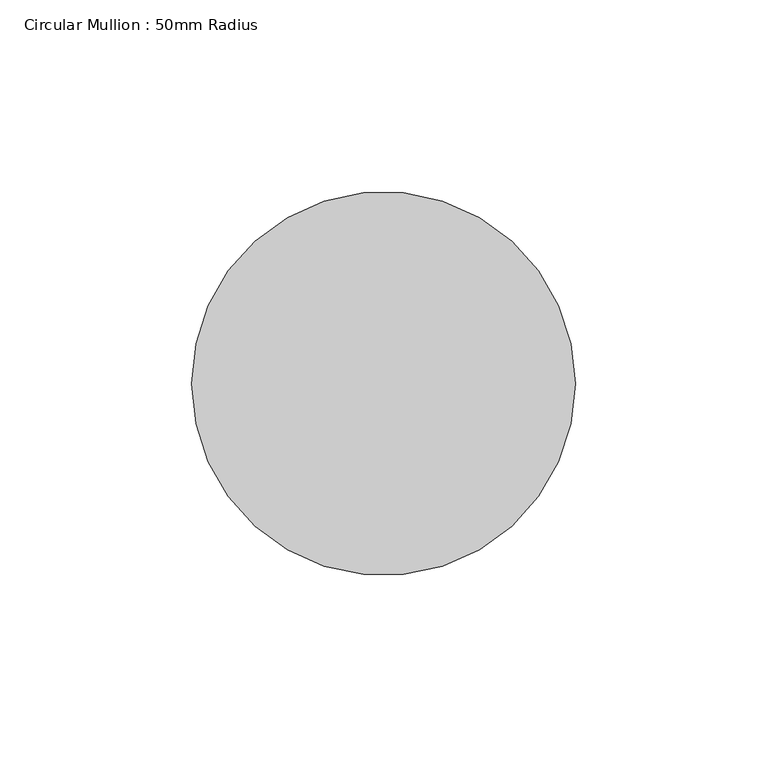
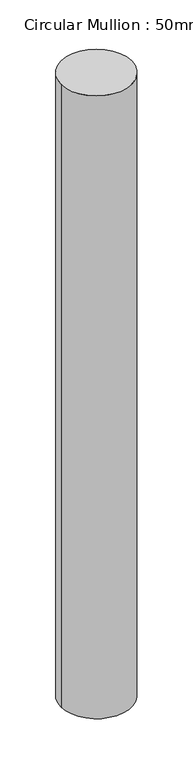
"""IFC4 building model written with IfcOpenShell, lengths in millimetres: member geometry, Circular Mullion : 50mm Radius."""

from ifc_helpers import new_model, si_unit, point, frame, origin, origin_2d, place, context, project, spatial, circle_curve, trimmed, segment, composite_curve, outline, extrude, source, transform, mapped, element, save


def circular_mullion_50mm_radius_791777ee(model_context):
    return source(origin(), model_context, "Body", "SweptSolid", [
        extrude(outline(composite_curve([segment(trimmed(circle_curve(origin_2d(), 50.0), [point((50.0, 0.0))], [point((-50.0, 0.0))], False, "CARTESIAN"), True, "CONTINUOUS"), segment(trimmed(circle_curve(origin_2d(), 50.0), [point((-50.0, 0.0))], [point((50.0, 0.0))], False, "CARTESIAN"), True, "CONTINUOUS")], self_intersect=False)), frame((0.0, 0.0, -933.617553), z_axis=(0.0, 0.0, 1.0), x_axis=(1.0, 0.0, 0.0)), (0.0, 0.0, 1.0), 933.617553),
    ])


if __name__ == "__main__":
    model = new_model("IFC4")
    model_context = context("Model", 3, world=origin())
    ifc_project = project(units=[si_unit("LENGTHUNIT", "METRE", prefix="MILLI")], contexts=[model_context])
    site = spatial("IfcSite", under=ifc_project)
    building = spatial("IfcBuilding", under=site)
    placement = place(None, origin())
    circular_mullion_50mm_radius_shape = circular_mullion_50mm_radius_791777ee(model_context)
    element("IfcMember", 1, ObjectType="Circular Mullion : 50mm Radius", at=placement, inside=building, context=model_context, shape_type="MappedRepresentation", body=[
        mapped(circular_mullion_50mm_radius_shape, transform((0.0, 0.0, 0.0), x_axis=(1.0, 0.0, 0.0), y_axis=(0.0, 1.0, 0.0), z_axis=(0.0, 0.0, 1.0))),
    ])
    save(model, "model.ifc")

# Revit data of these elements
# Type "Circular Mullion : 50mm Radius"
#   built-in parameter 1007350 = 0.164042 (stored number, unit not read)
# Element 1 (IfcMember, "Circular Mullion : 50mm Radius")
#   Materials on its faces: "Aluminium"
# Materials
#   "Aluminium": class "Metal", colour RGB 247 247 247, transparency 0, Description = "Aluminium 6061", Cost = 0
